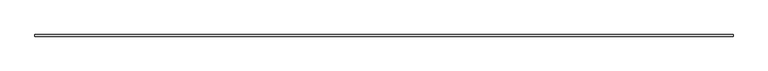
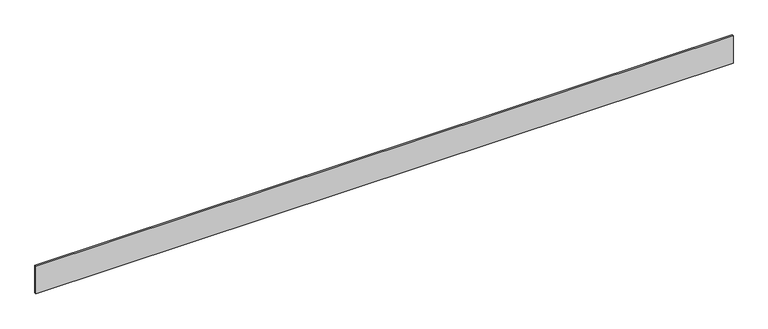
"""IFC4 building model written with IfcOpenShell, lengths in millimetres: proxy geometry, Inner panel:Inner panel:1:Inner panel:1 : Inner panel:Inner panel:300324:300043:Inner panel:1:Inner panel:1 : Inner panel:Inner panel:300324:300043 : Inner panel:Inner panel:1:Inner panel:1 : Inner panel:Inner panel:300324:300043:31 : Inner panel:Inner panel:1:Inner panel:1 : Inner panel:Inner panel:300324:300043:Inner panel:1:Inner panel:1 : Inner panel:Inner panel:300324:300043 : Inner panel:Inner panel:1:Inner panel:1 : Inner panel:Inner panel:300324:300043:300031."""

from ifc_helpers import new_model, si_unit, frame, origin, place, context, project, spatial, polyline, outline, extrude, source, transform, mapped, element, save


def generic_models_5e77d03c(model_context):
    return source(origin(), model_context, "Body", "SweptSolid", [
        extrude(outline(polyline([(562377.9746545, -578778.4413841), (570446.2867239, -578778.4413841), (570446.2867239, -578797.4913841), (562377.9746545, -578797.4913841), (562377.9746545, -578778.4413841)])), frame((0.0, 0.0, 3721.1), z_axis=(0.0, 0.0, 1.0), x_axis=(1.0, 0.0, 0.0)), (0.0, 0.0, 1.0), 336.5809035),
    ])


if __name__ == "__main__":
    model = new_model("IFC4")
    model_context = context("Model", 3, world=origin())
    ifc_project = project(units=[si_unit("LENGTHUNIT", "METRE", prefix="MILLI")], contexts=[model_context])
    site = spatial("IfcSite", under=ifc_project)
    building = spatial("IfcBuilding", under=site)
    placement = place(None, origin())
    generic_models_shape = generic_models_5e77d03c(model_context)
    element("IfcBuildingElementProxy", 1, Name="Inner panel:Inner panel:1:Inner panel:1 : Inner panel:Inner panel:300324:300043:Inner panel:1:Inner panel:1 : Inner panel:Inner panel:300324:300043 : Inner panel:Inner panel:1:Inner panel:1 : Inner panel:Inner panel:300324:300043:31 : Inner panel:Inner panel:1:Inner panel:1 : Inner panel:Inner panel:300324:300043:Inner panel:1:Inner panel:1 : Inner panel:Inner panel:300324:300043 : Inner panel:Inner panel:1:Inner panel:1 : Inner panel:Inner panel:300324:300043:300031", ObjectType="Inner panel:Inner panel:1:Inner panel:1 : Inner panel:Inner panel:300324:300043:Inner panel:1:Inner panel:1 : Inner panel:Inner panel:300324:300043 : Inner panel:Inner panel:1:Inner panel:1 : Inner panel:Inner panel:300324:300043:31 : Inner panel:Inner panel:1:Inner panel:1 : Inner panel:Inner panel:300324:300043:Inner panel:1:Inner panel:1 : Inner panel:Inner panel:300324:300043 : Inner panel:Inner panel:1:Inner panel:1 : Inner panel:Inner panel:300324:300043:300031", at=placement, inside=building, context=model_context, shape_type="MappedRepresentation", body=[
        mapped(generic_models_shape, transform((0.0, 0.0, 0.0), x_axis=(1.0, 0.0, 0.0), y_axis=(0.0, 1.0, 0.0), z_axis=(0.0, 0.0, 1.0))),
    ])
    save(model, "model.ifc")

# Revit data of these elements
# Type "Inner panel:Inner panel:1:Inner panel:1 : Inner panel:Inner panel:300324:300043:Inner panel:1:Inner panel:1 : Inner panel:Inner panel:300324:300043 : Inner panel:Inner panel:1:Inner panel:1 : Inner panel:Inner panel:300324:300043:31 : Inner panel:Inner panel:1:Inner panel:1 : Inner panel:Inner panel:300324:300043:Inner panel:1:Inner panel:1 : Inner panel:Inner panel:300324:300043 : Inner panel:Inner panel:1:Inner panel:1 : Inner panel:Inner panel:300324:300043:300031"
#   NameOverride = "Inner panel:Inner panel:1:Inner panel:1 : Inner panel:Inner panel:300324:300043:Inner panel:1:Inner panel:1 : Inner panel:Inner panel:300324:300043 : Inner panel:Inner panel:1:Inner panel:1 : Inner panel:Inner panel:300324:300043:300031"
#   ObjectTypeOverride = "Inner panel:1:Inner panel:1 : Inner panel:Inner panel:300324:300043 : Inner panel:Inner panel:1:Inner panel:1 : Inner panel:Inner panel:300324:300043"
#   Reference = "Inner panel"
#   Tag = "300031"
# Element 1 (IfcBuildingElementProxy, "Inner panel:Inner panel:1:Inner panel:1 : Inner panel:Inner panel:300324:300043:Inner panel:1:Inner panel:1 : Inner panel:Inner panel:300324:300043 : Inner panel:Inner panel:1:Inner panel:1 : Inner panel:Inner panel:300324:300043:31 : Inner panel:Inner panel:1:Inner panel:1 : Inner panel:Inner panel:300324:300043:Inner panel:1:Inner panel:1 : Inner panel:Inner panel:300324:300043 : Inner panel:Inner panel:1:Inner panel:1 : Inner panel:Inner panel:300324:300043:300031")
#   Materials on its faces: "¾” (CLASS A) FIRE RETARDANT PLYWOOD ...OR… IF 1/4\" GYP. BD UNDER PLYWOOD, FLAME SPREAD TO BE CLASS C -  (FINISH: GRADE B - PREFINISHED STAINED/SEALED) - 1/4\" GAP BTWN PANELS (FASTENERS T.B.D.)"
# Materials
#   "¾” (CLASS A) FIRE RETARDANT PLYWOOD ...OR… IF 1/4\" GYP. BD UNDER PLYWOOD, FLAME SPREAD TO BE CLASS C -  (FINISH: GRADE B - PREFINISHED STAINED/SEALED) - 1/4\" GAP BTWN PANELS (FASTENERS T.B.D.)": class "Wood", colour RGB 149 120 74, transparency 0, Description = "Plywood, sheathing grade", Cost = 0
